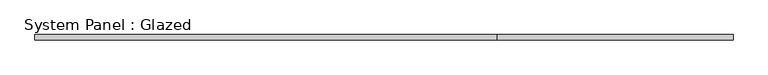
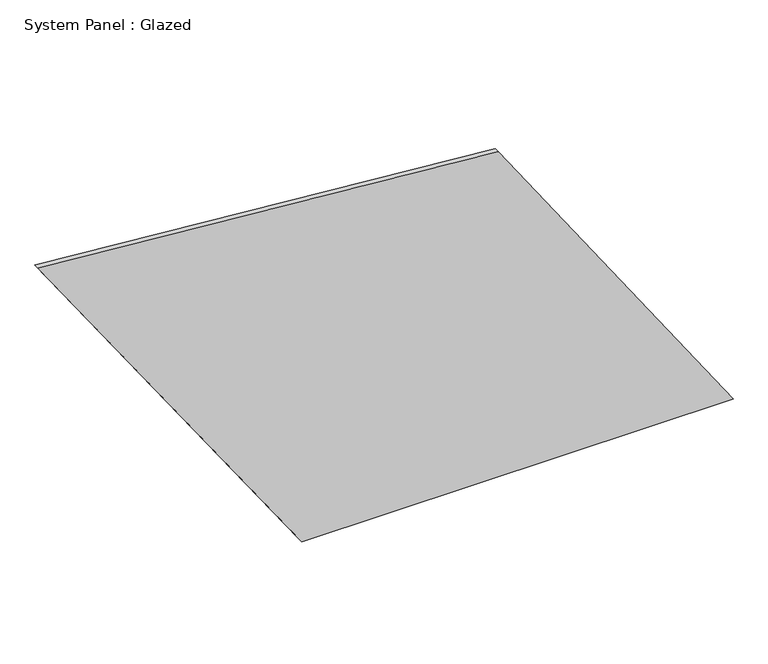
"""IFC4 building model written with IfcOpenShell, lengths in millimetres: plate geometry, System Panel : Glazed."""

import ifcopenshell
import ifcopenshell.guid

model = None  # the IFC model being written
_history = None  # IfcOwnerHistory: only IFC2X3 demands one
_inside = {}  # id of a spatial element -> (the spatial element, [elements in it])
_under = {}  # id of a project, library or spatial element -> (it, [spatial elements below it])
_declared = {}  # id of a project -> (the project, [libraries it declares])
_typed = {}  # id of a type object -> (the type object, [elements of that type])
_made_of = {}  # id of a material, layer set ... -> (it, [elements and type objects made of it])


def new_model(schema):
    """Start an empty IFC model of exactly this schema.

    Asked for "IFC4X3", IfcOpenShell would pick the latest addendum, in which some entities
    have other attributes; the version numbers below select the first issue.
    IFC2X3 requires an IfcOwnerHistory on every rooted entity: one is made here for all.
    """
    global model, _history
    if schema == "IFC4X3":
        model = ifcopenshell.file(schema_version=(4, 3, 0, 0))
    else:
        model = ifcopenshell.file(schema=schema)
    _inside.clear()
    _under.clear()
    _declared.clear()
    _typed.clear()
    _made_of.clear()
    _history = None
    if model.schema == "IFC2X3":
        org = make("IfcOrganization", Name="unknown")
        user = make(
            "IfcPersonAndOrganization",
            ThePerson=make("IfcPerson", FamilyName="unknown"),
            TheOrganization=org,
        )
        app = make(
            "IfcApplication",
            ApplicationDeveloper=org,
            Version="unknown",
            ApplicationFullName="unknown",
            ApplicationIdentifier="unknown",
        )
        _history = make(
            "IfcOwnerHistory",
            OwningUser=user,
            OwningApplication=app,
            ChangeAction="ADDED",
            CreationDate=0,
        )
    return model


def make(cls, **values):
    """One entity of the class cls with the attributes given. An attribute that is None is left unset."""
    return model.create_entity(
        cls, **{name: value for name, value in values.items() if value is not None}
    )


def rooted(cls, **values):
    """An entity with a GlobalId (a new one), such as an element, a storey or a relation."""
    return make(cls, GlobalId=ifcopenshell.guid.new(), OwnerHistory=_history, **values)


def si_unit(unit_type, name, prefix=None):
    """IfcSIUnit, for example si_unit("LENGTHUNIT", "METRE", prefix="MILLI")."""
    return make("IfcSIUnit", UnitType=unit_type, Prefix=prefix, Name=name)


def assignment(units):
    """IfcUnitAssignment: the units of a project."""
    return None if units is None else make("IfcUnitAssignment", Units=units)


def point(xyz):
    """IfcCartesianPoint."""
    return None if xyz is None else make("IfcCartesianPoint", Coordinates=xyz)


def direction(xyz):
    """IfcDirection."""
    return None if xyz is None else make("IfcDirection", DirectionRatios=xyz)


def frame(location, z_axis=None, x_axis=None):
    """IfcAxis2Placement3D, a coordinate frame: its origin and axes. An axis left out is left unset."""
    return make(
        "IfcAxis2Placement3D",
        Location=point(location),
        Axis=direction(z_axis),
        RefDirection=direction(x_axis),
    )


def origin():
    """The frame at (0, 0, 0) with its axes left unset."""
    return frame((0.0, 0.0, 0.0))


def place(relative_to, where):
    """IfcLocalPlacement: puts the frame where relative to a parent placement (None: the world)."""
    return make(
        "IfcLocalPlacement", PlacementRelTo=relative_to, RelativePlacement=where
    )


def context(
    kind, dimensions, precision=None, world=None, true_north=None, identifier=None
):
    """IfcGeometricRepresentationContext, for example the 3D "Model" context."""
    return make(
        "IfcGeometricRepresentationContext",
        ContextIdentifier=identifier,
        ContextType=kind,
        CoordinateSpaceDimension=dimensions,
        Precision=precision,
        WorldCoordinateSystem=world,
        TrueNorth=true_north,
    )


def project(units=None, contexts=None):
    """IfcProject with its units and contexts."""
    return rooted(
        "IfcProject",
        Name="project",
        RepresentationContexts=contexts,
        UnitsInContext=assignment(units),
    )


def spatial(cls, under=None, at=None, **own):
    """A site, building, storey or space (cls), placed at a placement, below another one or the project."""
    s = rooted(cls, ObjectPlacement=at, **own)
    if under is not None:
        _under.setdefault(under.id(), (under, []))[1].append(s)
    return s


def polyline(points):
    """IfcPolyline through the points."""
    return make("IfcPolyline", Points=[point(p) for p in points])


def outline(outer, holes=None, kind="AREA"):
    """IfcArbitraryClosedProfileDef: a profile drawn as a closed curve; with holes, ...WithVoids."""
    if holes is None:
        return make("IfcArbitraryClosedProfileDef", ProfileType=kind, OuterCurve=outer)
    return make(
        "IfcArbitraryProfileDefWithVoids",
        ProfileType=kind,
        OuterCurve=outer,
        InnerCurves=holes,
    )


def extrude(swept, where, along, depth):
    """IfcExtrudedAreaSolid: the profile swept, set in the frame where, extruded along a direction by depth."""
    return make(
        "IfcExtrudedAreaSolid",
        SweptArea=swept,
        Position=where,
        ExtrudedDirection=direction(along),
        Depth=depth,
    )


def shape(context_of_items, identifier, shape_type, items):
    """IfcShapeRepresentation: the items that make up one representation, for example the "Body"."""
    return make(
        "IfcShapeRepresentation",
        ContextOfItems=context_of_items,
        RepresentationIdentifier=identifier,
        RepresentationType=shape_type,
        Items=items,
    )


def source(mapping_origin, context_of_items, identifier, shape_type, items):
    """IfcRepresentationMap: a shape defined once, which mapped items show again and again."""
    return make(
        "IfcRepresentationMap",
        MappingOrigin=mapping_origin,
        MappedRepresentation=shape(context_of_items, identifier, shape_type, items),
    )


def transform(
    local_origin,
    x_axis=None,
    y_axis=None,
    z_axis=None,
    scale=None,
    scale2=None,
    scale3=None,
    uniform=True,
):
    """IfcCartesianTransformationOperator3D, or its non-uniform kind. x_axis, y_axis, z_axis: its Axis1, 2, 3."""
    if uniform:
        return make(
            "IfcCartesianTransformationOperator3D",
            Axis1=direction(x_axis),
            Axis2=direction(y_axis),
            LocalOrigin=point(local_origin),
            Scale=scale,
            Axis3=direction(z_axis),
        )
    return make(
        "IfcCartesianTransformationOperator3DnonUniform",
        Axis1=direction(x_axis),
        Axis2=direction(y_axis),
        LocalOrigin=point(local_origin),
        Scale=scale,
        Axis3=direction(z_axis),
        Scale2=scale2,
        Scale3=scale3,
    )


def mapped(mapping_source, mapping_target):
    """IfcMappedItem: shows the shape of a source again, moved by a transform."""
    return make(
        "IfcMappedItem", MappingSource=mapping_source, MappingTarget=mapping_target
    )


def made_of(thing, what):
    """Note that an element or type object is made of a material, layer set ...; save() writes the relation."""
    if what is not None:
        _made_of.setdefault(what.id(), (what, []))[1].append(thing)
    return thing


def element(
    cls,
    number,
    at=None,
    inside=None,
    cuts=None,
    type_object=None,
    material=None,
    context=None,
    identifier="Body",
    shape_type=None,
    held_by="IfcProductDefinitionShape",
    body=None,
    shapes=None,
    **own,
):
    """One element of the class cls, such as IfcWall. Its Tag is "e" and its number.

    at: its placement. inside: the storey or other place that contains it. cuts: it is an
    opening in that element (IfcRelVoidsElement). A single representation is given by context,
    identifier, shape_type and body (its items); several are given by shapes. held_by: the class
    of the entity that holds the representations. save() writes the other relations.
    """
    e = rooted(cls, Tag="e%d" % number, ObjectPlacement=at, **own)
    if body is not None:
        shapes = [shape(context, identifier, shape_type, body)]
    if shapes is not None:
        e.Representation = make(held_by, Representations=shapes)
    if inside is not None:
        _inside.setdefault(inside.id(), (inside, []))[1].append(e)
    if cuts is not None:
        rooted(
            "IfcRelVoidsElement", RelatingBuildingElement=cuts, RelatedOpeningElement=e
        )
    if type_object is not None:
        _typed.setdefault(type_object.id(), (type_object, []))[1].append(e)
    return made_of(e, material)


def aggregate(whole, parts):
    """IfcRelAggregates: a whole, such as a stair, and the parts it consists of."""
    return rooted("IfcRelAggregates", RelatingObject=whole, RelatedObjects=parts)


def save(model, path):
    """Write the relations noted so far, then the file.

    IfcRelAggregates (storeys below a building ...), IfcRelContainedInSpatialStructure (elements
    in a storey), IfcRelDefinesByType, IfcRelAssociatesMaterial and IfcRelDeclares: one each for
    every whole, place, type object, material and project.
    """
    for whole, parts in _under.values():
        aggregate(whole, parts)
    for where, things in _inside.values():
        rooted(
            "IfcRelContainedInSpatialStructure",
            RelatedElements=things,
            RelatingStructure=where,
        )
    for kind, things in _typed.values():
        rooted("IfcRelDefinesByType", RelatedObjects=things, RelatingType=kind)
    for what, things in _made_of.values():
        rooted("IfcRelAssociatesMaterial", RelatedObjects=things, RelatingMaterial=what)
    for by, libraries in _declared.values():
        rooted("IfcRelDeclares", RelatingContext=by, RelatedDefinitions=libraries)
    model.write(path)


def system_panel_glazed_439fd929(model_context):
    return source(origin(), model_context, "Body", "SweptSolid", [
        extrude(outline(polyline([(0.0, -409.3038222), (0.0, 1699.402519), (1681.956178, 551.0807367), (1868.429734, -1699.402519), (0.0, -409.3038222)])), frame((0.0, -49.5, 0.0), z_axis=(0.0, 1.0, 0.0), x_axis=(0.0, 0.0, 1.0)), (0.0, 0.0, 1.0), 25.0),
    ])


if __name__ == "__main__":
    model = new_model("IFC4")
    model_context = context("Model", 3, world=origin())
    ifc_project = project(units=[si_unit("LENGTHUNIT", "METRE", prefix="MILLI")], contexts=[model_context])
    site = spatial("IfcSite", under=ifc_project)
    building = spatial("IfcBuilding", under=site)
    placement = place(None, origin())
    system_panel_glazed_shape = system_panel_glazed_439fd929(model_context)
    element("IfcPlate", 1, ObjectType="System Panel : Glazed", at=placement, inside=building, context=model_context, shape_type="MappedRepresentation", body=[
        mapped(system_panel_glazed_shape, transform((0.0, 0.0, 0.0), x_axis=(1.0, 0.0, 0.0), y_axis=(0.0, 1.0, 0.0), z_axis=(0.0, 0.0, 1.0))),
    ])
    save(model, "model.ifc")

# Revit data of these elements
# Element 1 (IfcPlate, "System Panel : Glazed")
#   Materials on its faces: "Glass, Clear Glazing"
# Materials
#   "Glass, Clear Glazing": class "Glass", colour RGB 247 249 248, transparency 0.85, Description = "Clear glazing", Cost = 0
